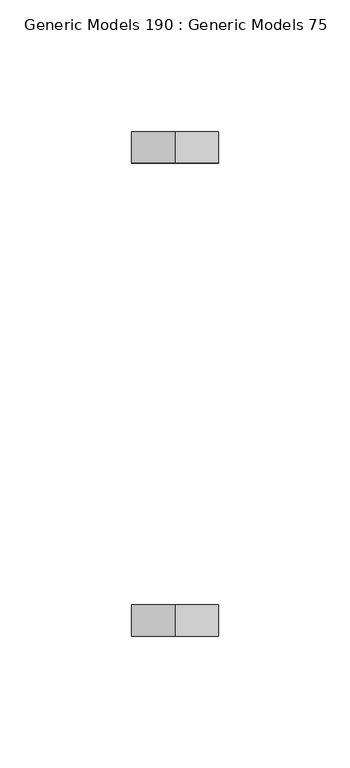
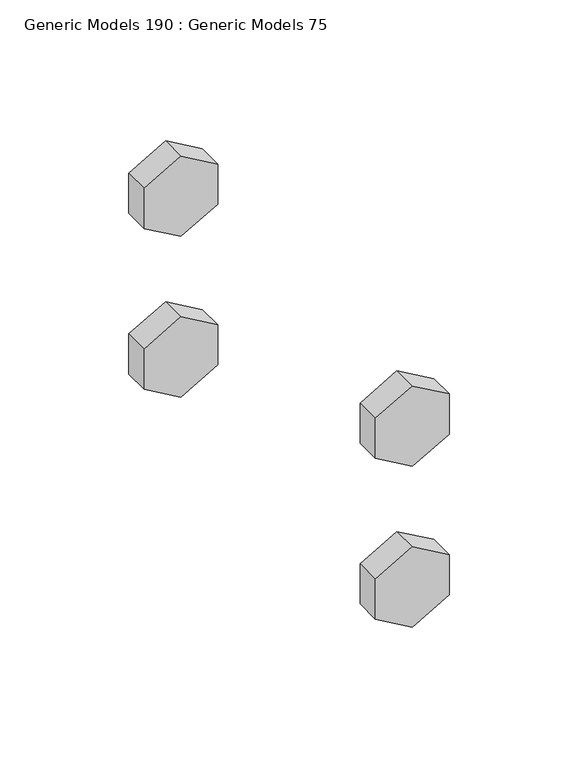
"""IFC4 building model written with IfcOpenShell, lengths in millimetres: proxy geometry, Generic Models 190 : Generic Models 75."""

from ifc_helpers import new_model, si_unit, frame, origin, place, context, project, spatial, polyline, outline, extrude, source, transform, mapped, element, save


def generic_models_190_generic_models_75_51f8eee1(model_context):
    return source(origin(), model_context, "Body", "SweptSolid", [
        extrude(outline(polyline([(271333.9125, 31991.9073871), (271352.9625, 31991.9073871), (271362.4875, 31975.4096032), (271352.9625, 31958.9118192), (271333.9125, 31958.9118192), (271324.3875, 31975.4096032), (271333.9125, 31991.9073871)])), frame((0.0, 30858.4781612, 0.0), z_axis=(0.0, 1.0, 0.0), x_axis=(0.0, 0.0, 1.0)), (0.0, 0.0, 1.0), 11.90625),
        extrude(outline(polyline([(271257.7125, 31991.9073871), (271276.7625, 31991.9073871), (271286.2875, 31975.4096032), (271276.7625, 31958.9118192), (271257.7125, 31958.9118192), (271248.1875, 31975.4096032), (271257.7125, 31991.9073871)])), frame((0.0, 30858.4781612, 0.0), z_axis=(0.0, 1.0, 0.0), x_axis=(0.0, 0.0, 1.0)), (0.0, 0.0, 1.0), 11.90625),
        extrude(outline(polyline([(271333.9125, 31991.9073871), (271352.9625, 31991.9073871), (271362.4875, 31975.4096032), (271352.9625, 31958.9118192), (271333.9125, 31958.9118192), (271324.3875, 31975.4096032), (271333.9125, 31991.9073871)])), frame((0.0, 30678.6937862, 0.0), z_axis=(0.0, 1.0, 0.0), x_axis=(0.0, 0.0, 1.0)), (0.0, 0.0, 1.0), 11.90625),
        extrude(outline(polyline([(271257.7125, 31991.9073871), (271276.7625, 31991.9073871), (271286.2875, 31975.4096032), (271276.7625, 31958.9118192), (271257.7125, 31958.9118192), (271248.1875, 31975.4096032), (271257.7125, 31991.9073871)])), frame((0.0, 30678.6937862, 0.0), z_axis=(0.0, 1.0, 0.0), x_axis=(0.0, 0.0, 1.0)), (0.0, 0.0, 1.0), 11.90625),
    ])


if __name__ == "__main__":
    model = new_model("IFC4")
    model_context = context("Model", 3, world=origin())
    ifc_project = project(units=[si_unit("LENGTHUNIT", "METRE", prefix="MILLI")], contexts=[model_context])
    site = spatial("IfcSite", under=ifc_project)
    building = spatial("IfcBuilding", under=site)
    placement = place(None, origin())
    generic_models_190_generic_models_75_shape = generic_models_190_generic_models_75_51f8eee1(model_context)
    element("IfcBuildingElementProxy", 1, Name="Generic Models 190 : Generic Models 75", ObjectType="Generic Models 190 : Generic Models 75", at=placement, inside=building, context=model_context, shape_type="MappedRepresentation", body=[
        mapped(generic_models_190_generic_models_75_shape, transform((0.0, 0.0, 0.0), x_axis=(1.0, 0.0, 0.0), y_axis=(0.0, 1.0, 0.0), z_axis=(0.0, 0.0, 1.0))),
    ])
    save(model, "model.ifc")
